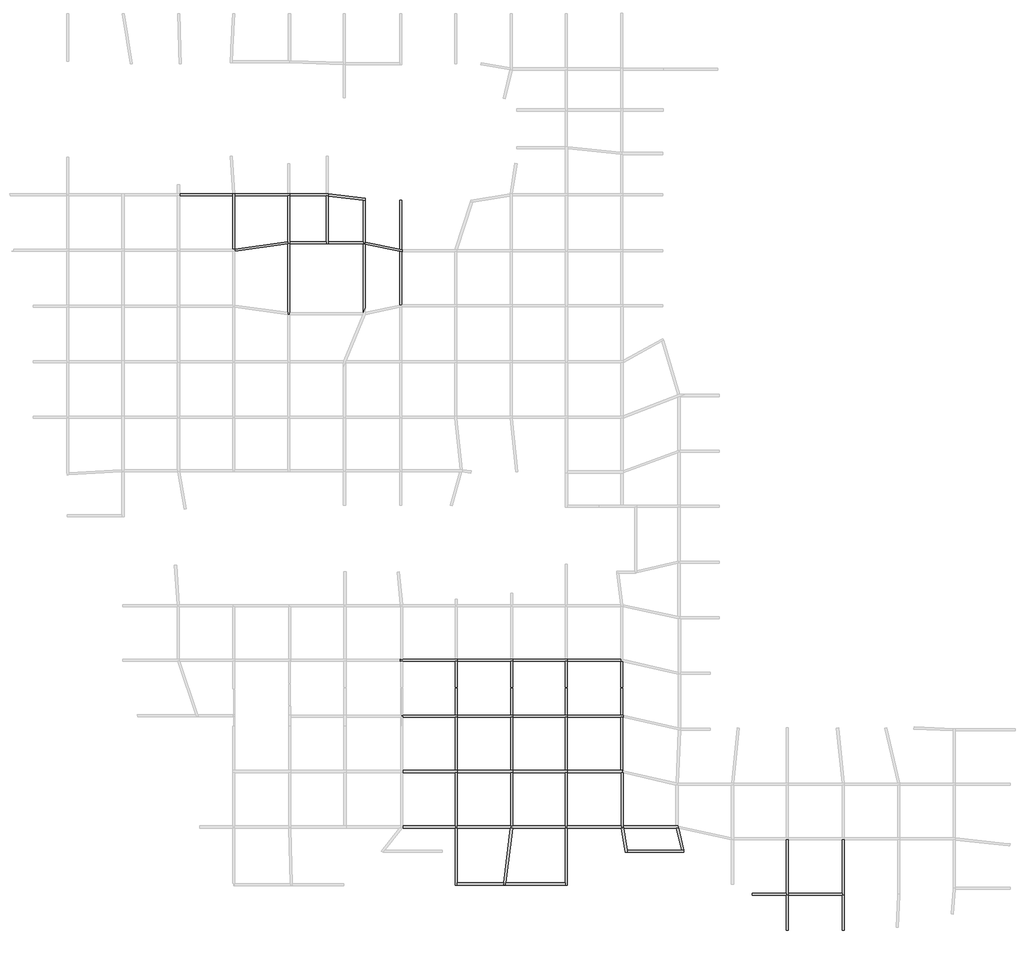
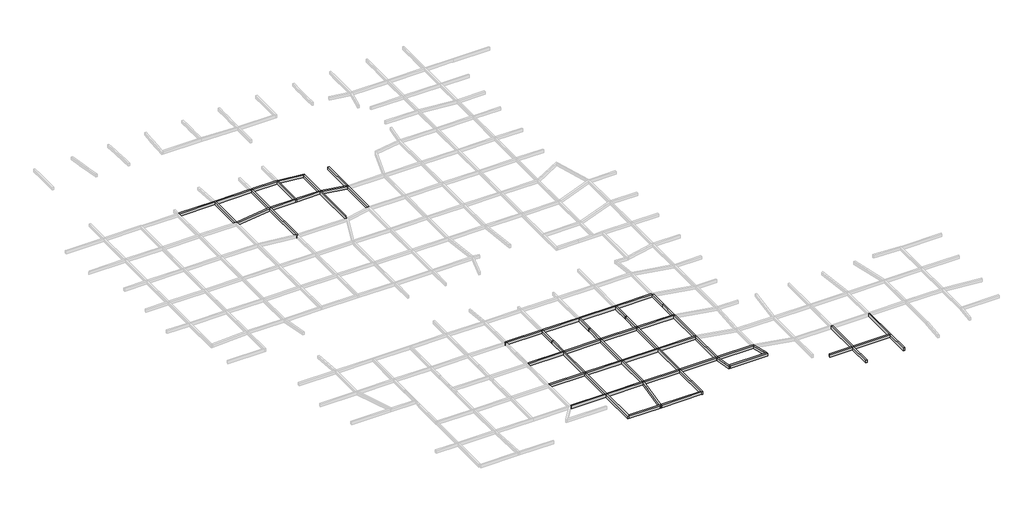
# One storey, part 3 of 8: 59 beams.
"""IFC4 building model written with IfcOpenShell, lengths in millimetres."""

from ifc_helpers import new_model, si_unit, frame, origin, place, context, project, spatial, polyline, outline, extrude, faceted_brep, element, save

model = new_model("IFC4")

# Units and contexts
model_context = context("Model", 3, world=origin())
ifc_project = project(units=[si_unit("LENGTHUNIT", "METRE", prefix="MILLI")], contexts=[model_context])

# Site, building, storey
site = spatial("IfcSite", under=ifc_project)
building = spatial("IfcBuilding", under=site)
storey = spatial("IfcBuildingStorey", under=building, Name="层高", Elevation=3300.0)

# Beams
placement = place(None, origin())
element("IfcBeam", 1, ObjectType="混凝土 - 矩形梁 : KL_beam", at=placement, inside=storey, context=model_context, shape_type="Brep", body=[
    faceted_brep([(101970.8225114, 127335.802002, 3300.0), (101960.6997743, 127335.802002, 3300.0), (101670.8225114, 127335.802002, 3300.0), (101670.8225114, 127035.802002, 3300.0), (101670.8225114, 119435.802002, 3300.0), (101970.8225114, 119435.802002, 3300.0), (101970.8225114, 119458.440122, 3300.0), (101970.8225114, 127035.802002, 3300.0), (101970.8225114, 127191.0401174, 3300.0), (101970.8225114, 127335.802002, 2700.0), (101970.8225114, 119435.802002, 2700.0), (101970.8225114, 119458.440122, 2700.0), (101970.8225114, 127035.802002, 2700.0), (101970.8225114, 127191.0401174, 2700.0), (101670.8225114, 127335.802002, 2700.0), (101960.6997743, 127335.802002, 2700.0), (101670.8225114, 119435.802002, 2700.0), (101670.8225114, 127035.802002, 2700.0)], [[[0, 1, 2, 3, 4, 5, 6, 7, 8]], [[9, 0, 8, 7, 6, 5, 10, 11, 12, 13]], [[14, 15, 9, 13, 12, 11, 10, 16, 17]], [[2, 14, 17, 16, 4, 3]], [[5, 4, 16, 10]], [[2, 1, 0, 9, 15, 14]]]),
])
element("IfcBeam", 2, ObjectType="混凝土 - 矩形梁 : KL_beam", at=placement, inside=storey, context=model_context, shape_type="Brep", body=[
    faceted_brep([(94070.8225114, 127335.802002, 3300.0), (94070.8225114, 127035.802002, 3300.0), (101670.8225114, 127035.802002, 3300.0), (101670.8225114, 127335.802002, 3300.0), (101659.9672049, 127335.802002, 3300.0), (94070.8225114, 127035.802002, 2700.0), (101670.8225114, 127035.802002, 2700.0), (94070.8225114, 127335.802002, 2700.0), (101659.9672049, 127335.802002, 2700.0), (101670.8225114, 127335.802002, 2700.0)], [[[0, 1, 2, 3, 4]], [[1, 5, 6, 2]], [[5, 7, 8, 9, 6]], [[7, 0, 4, 3, 9, 8]], [[1, 0, 7, 5]], [[3, 2, 6, 9]]]),
])
element("IfcBeam", 3, ObjectType="混凝土 - 矩形梁 : KL_beam", at=placement, inside=storey, context=model_context, shape_type="Brep", body=[
    faceted_brep([(109770.8225114, 127035.802002, 3300.0), (109770.8225114, 127335.802002, 3300.0), (109470.8225114, 127335.802002, 3300.0), (101970.8225114, 127335.802002, 3300.0), (101970.8225114, 127191.0401174, 3300.0), (101981.6778179, 127035.802002, 3300.0), (109470.8225114, 127035.802002, 3300.0), (109770.8225114, 127035.802002, 2700.0), (101981.6778179, 127035.802002, 2700.0), (109470.8225114, 127035.802002, 2700.0), (109770.8225114, 127335.802002, 2700.0), (101970.8225114, 127191.0401174, 2700.0), (101970.8225114, 127335.802002, 2700.0), (109470.8225114, 127335.802002, 2700.0)], [[[0, 1, 2, 3, 4, 5, 6]], [[7, 0, 6, 5, 8, 9]], [[10, 7, 9, 8, 11, 12, 13]], [[12, 3, 2, 1, 10, 13]], [[3, 12, 11, 4]], [[5, 4, 11, 8]], [[1, 0, 7, 10]]]),
])
element("IfcBeam", 4, ObjectType="混凝土 - 矩形梁 : KL_beam", at=placement, inside=storey, context=model_context, shape_type="Brep", body=[
    faceted_brep([(115273.8238915, 127035.802002, 3300.0), (115273.8238915, 127318.5107917, 3300.0), (115273.8238915, 127335.802002, 3300.0), (114973.8238915, 127335.802002, 3300.0), (109770.8225114, 127335.802002, 3300.0), (109770.8225114, 127035.802002, 3300.0), (114973.8238915, 127035.802002, 3300.0), (115114.6494985, 127035.802002, 3300.0), (115273.8238915, 127035.802002, 2700.0), (109770.8225114, 127035.802002, 2700.0), (114973.8238915, 127035.802002, 2700.0), (115114.6494985, 127035.802002, 2700.0), (115273.8238915, 127335.802002, 2700.0), (115273.8238915, 127318.5107917, 2700.0), (109770.8225114, 127335.802002, 2700.0), (114973.8238915, 127335.802002, 2700.0)], [[[0, 1, 2, 3, 4, 5, 6, 7]], [[8, 0, 7, 6, 5, 9, 10, 11]], [[12, 13, 8, 11, 10, 9, 14, 15]], [[2, 12, 15, 14, 4, 3]], [[5, 4, 14, 9]], [[2, 1, 0, 8, 13, 12]]]),
])
element("IfcBeam", 5, ObjectType="混凝土 - 矩形梁 : KL_beam", at=placement, inside=storey, context=model_context, shape_type="Brep", body=[
    faceted_brep([(115273.8238915, 127035.802002, 3300.0), (115114.6494985, 127035.802002, 3300.0), (115273.8238915, 127016.2578441, 3300.0), (120234.3184952, 126407.1856923, 3300.0), (120534.3184952, 126370.350324, 3300.0), (120534.3184952, 126672.6032717, 3300.0), (115273.8238915, 127318.5107917, 3300.0), (115114.6494985, 127035.802002, 2700.0), (115273.8238915, 127016.2578441, 2700.0), (120234.3184952, 126407.1856923, 2700.0), (120534.3184952, 126370.350324, 2700.0), (115273.8238915, 127035.802002, 2700.0), (115273.8238915, 127318.5107917, 2700.0), (120534.3184952, 126672.6032717, 2700.0)], [[[0, 1, 2, 3, 4, 5, 6]], [[1, 7, 8, 9, 10, 4, 3, 2]], [[7, 11, 12, 13, 10, 9, 8]], [[12, 6, 5, 13]], [[0, 11, 7, 1]], [[11, 0, 6, 12]], [[5, 4, 10, 13]]]),
])
element("IfcBeam", 6, ObjectType="混凝土 - 矩形梁 : KL_beam", at=placement, inside=storey, context=model_context, shape_type="Brep", body=[
    faceted_brep([(109470.8225114, 120235.802002, 3300.0), (109770.8225114, 120235.802002, 3300.0), (109770.8225114, 120535.802002, 3300.0), (109770.8225114, 127035.802002, 3300.0), (109470.8225114, 127035.802002, 3300.0), (109470.8225114, 120516.1324297, 3300.0), (109470.8225114, 120235.802002, 2700.0), (109470.8225114, 127035.802002, 2700.0), (109470.8225114, 120516.1324297, 2700.0), (109770.8225114, 120235.802002, 2700.0), (109770.8225114, 127035.802002, 2700.0), (109770.8225114, 120535.802002, 2700.0)], [[[0, 1, 2, 3, 4, 5]], [[6, 0, 5, 4, 7, 8]], [[9, 6, 8, 7, 10, 11]], [[1, 9, 11, 10, 3, 2]], [[4, 3, 10, 7]], [[1, 0, 6, 9]]]),
])
element("IfcBeam", 7, ObjectType="混凝土 - 矩形梁 : KL_beam", at=placement, inside=storey, context=model_context, shape_type="Brep", body=[
    faceted_brep([(109470.8225114, 110106.8473936, 3300.0), (109770.8225114, 110106.8473936, 3300.0), (109770.8225114, 110406.8473936, 3300.0), (109770.8225114, 120235.802002, 3300.0), (109470.8225114, 120235.802002, 3300.0), (109470.8225114, 120213.1638821, 3300.0), (109470.8225114, 110428.8334253, 3300.0), (109470.8225114, 110126.0228157, 3300.0), (109470.8225114, 110106.8473936, 2700.0), (109470.8225114, 120235.802002, 2700.0), (109470.8225114, 120213.1638821, 2700.0), (109470.8225114, 110428.8334253, 2700.0), (109470.8225114, 110126.0228157, 2700.0), (109770.8225114, 110106.8473936, 2700.0), (109770.8225114, 120235.802002, 2700.0), (109770.8225114, 110406.8473936, 2700.0)], [[[0, 1, 2, 3, 4, 5, 6, 7]], [[8, 0, 7, 6, 5, 4, 9, 10, 11, 12]], [[13, 8, 12, 11, 10, 9, 14, 15]], [[1, 13, 15, 14, 3, 2]], [[4, 3, 14, 9]], [[1, 0, 8, 13]]]),
])
element("IfcBeam", 8, ObjectType="混凝土 - 矩形梁 : KL_beam", at=placement, inside=storey, context=model_context, shape_type="Brep", body=[
    faceted_brep([(114973.8238915, 120235.802002, 3300.0), (115273.8238915, 120235.802002, 3300.0), (115273.8238915, 120535.802002, 3300.0), (115273.8238915, 127016.2578441, 3300.0), (115114.6494985, 127035.802002, 3300.0), (114973.8238915, 127035.802002, 3300.0), (114973.8238915, 120535.802002, 3300.0), (114973.8238915, 127035.802002, 2700.0), (114973.8238915, 120535.802002, 2700.0), (114973.8238915, 120235.802002, 2700.0), (115273.8238915, 120235.802002, 2700.0), (115114.6494985, 127035.802002, 2700.0), (115273.8238915, 127016.2578441, 2700.0), (115273.8238915, 120535.802002, 2700.0)], [[[0, 1, 2, 3, 4, 5, 6]], [[5, 7, 8, 9, 0, 6]], [[10, 9, 8, 7, 11, 12, 13]], [[1, 10, 13, 12, 3, 2]], [[7, 5, 4, 11]], [[4, 3, 12, 11]], [[1, 0, 9, 10]]]),
])
element("IfcBeam", 9, ObjectType="混凝土 - 矩形梁 : KL_beam", at=placement, inside=storey, context=model_context, shape_type="Brep", body=[
    faceted_brep([(120234.3184952, 120235.802002, 3300.0), (120534.3184952, 120235.802002, 3300.0), (120534.3184952, 120466.4709981, 3300.0), (120534.3184952, 126370.350324, 3300.0), (120234.3184952, 126407.1856923, 3300.0), (120234.3184952, 120535.802002, 3300.0), (120234.3184952, 120235.802002, 2700.0), (120234.3184952, 126407.1856923, 2700.0), (120234.3184952, 120535.802002, 2700.0), (120534.3184952, 120235.802002, 2700.0), (120534.3184952, 126370.350324, 2700.0), (120534.3184952, 120466.4709981, 2700.0)], [[[0, 1, 2, 3, 4, 5]], [[6, 0, 5, 4, 7, 8]], [[9, 6, 8, 7, 10, 11]], [[1, 9, 11, 10, 3, 2]], [[4, 3, 10, 7]], [[1, 0, 6, 9]]]),
])
element("IfcBeam", 10, ObjectType="混凝土 - 矩形梁 : KL_beam", at=placement, inside=storey, context=model_context, shape_type="SweptSolid", body=[
    extrude(outline(polyline([(109770.8225114, 120235.802002), (109770.8225114, 120535.802002), (114973.8238915, 120535.802002), (114973.8238915, 120235.802002), (109770.8225114, 120235.802002)])), frame((0.0, 0.0, 2700.0), z_axis=(0.0, 0.0, 1.0), x_axis=(1.0, 0.0, 0.0)), (0.0, 0.0, 1.0), 600.0),
])
element("IfcBeam", 11, ObjectType="混凝土 - 矩形梁 : KL_beam", at=placement, inside=storey, context=model_context, shape_type="SweptSolid", body=[
    extrude(outline(polyline([(115273.8238915, 120235.802002), (115273.8238915, 120535.802002), (120234.3184952, 120535.802002), (120234.3184952, 120235.802002), (115273.8238915, 120235.802002)])), frame((0.0, 0.0, 2700.0), z_axis=(0.0, 0.0, 1.0), x_axis=(1.0, 0.0, 0.0)), (0.0, 0.0, 1.0), 600.0),
])
element("IfcBeam", 12, ObjectType="混凝土 - 矩形梁 : KL_beam", at=placement, inside=storey, context=model_context, shape_type="Brep", body=[
    faceted_brep([(120234.3184952, 110286.2989162, 3300.0), (120534.3184952, 111020.8146845, 3300.0), (120534.3184952, 120159.7688197, 3300.0), (120234.3184952, 120223.5357882, 3300.0), (120234.3184952, 110406.8473936, 3300.0), (120234.3184952, 110286.2989162, 2700.0), (120234.3184952, 120223.5357882, 2700.0), (120234.3184952, 110406.8473936, 2700.0), (120534.3184952, 111020.8146845, 2700.0), (120534.3184952, 120159.7688197, 2700.0)], [[[0, 1, 2, 3, 4]], [[5, 0, 4, 3, 6, 7]], [[8, 5, 7, 6, 9]], [[1, 8, 9, 2]], [[1, 0, 5, 8]], [[3, 2, 9, 6]]]),
])
element("IfcBeam", 13, ObjectType="混凝土 - 矩形梁 : KL_beam", at=placement, inside=storey, context=model_context, shape_type="Brep", body=[
    faceted_brep([(120234.3184952, 120223.5357882, 3300.0), (120534.3184952, 120159.7688197, 3300.0), (125448.8238726, 119115.1584543, 3300.0), (125748.8238726, 119051.3914858, 3300.0), (125783.0582452, 119044.1147453, 3300.0), (125814.5895158, 119344.1147453, 3300.0), (125748.8238726, 119358.0936643, 3300.0), (125448.8238726, 119421.8606328, 3300.0), (120534.3184952, 120466.4709981, 3300.0), (120534.3184952, 120235.802002, 3300.0), (120234.3184952, 120235.802002, 3300.0), (120234.3184952, 120223.5357882, 2700.0), (120534.3184952, 120159.7688197, 2700.0), (125448.8238726, 119115.1584543, 2700.0), (125748.8238726, 119051.3914858, 2700.0), (125783.0582452, 119044.1147453, 2700.0), (120234.3184952, 120235.802002, 2700.0), (120534.3184952, 120235.802002, 2700.0), (120534.3184952, 120466.4709981, 2700.0), (125448.8238726, 119421.8606328, 2700.0), (125748.8238726, 119358.0936643, 2700.0), (125814.5895158, 119344.1147453, 2700.0)], [[[0, 1, 2, 3, 4, 5, 6, 7, 8, 9, 10]], [[4, 3, 2, 1, 0, 11, 12, 13, 14, 15]], [[15, 14, 13, 12, 11, 16, 17, 18, 19, 20, 21]], [[8, 7, 6, 5, 21, 20, 19, 18]], [[11, 0, 10, 16]], [[9, 17, 16, 10]], [[17, 9, 8, 18]], [[5, 4, 15, 21]]]),
])
element("IfcBeam", 14, ObjectType="混凝土 - 矩形梁 : KL_beam", at=placement, inside=storey, context=model_context, shape_type="SweptSolid", body=[
    extrude(outline(polyline([(125748.8238726, 111550.4593009), (125448.8238726, 111486.6923324), (125448.8238726, 119115.1584543), (125748.8238726, 119051.3914858), (125748.8238726, 111550.4593009)])), frame((0.0, 0.0, 2700.0), z_axis=(0.0, 0.0, 1.0), x_axis=(1.0, 0.0, 0.0)), (0.0, 0.0, 1.0), 600.0),
])
element("IfcBeam", 15, ObjectType="混凝土 - 矩形梁 : KL_beam", at=placement, inside=storey, context=model_context, shape_type="SweptSolid", body=[
    extrude(outline(polyline([(125448.8238726, 126395.9353335), (125748.8238726, 126395.9353335), (125748.8238726, 119358.0936643), (125448.8238726, 119421.8606328), (125448.8238726, 126395.9353335)])), frame((0.0, 0.0, 2700.0), z_axis=(0.0, 0.0, 1.0), x_axis=(1.0, 0.0, 0.0)), (0.0, 0.0, 1.0), 600.0),
])
element("IfcBeam", 16, ObjectType="混凝土 - 矩形梁 : KL_beam", at=placement, inside=storey, context=model_context, shape_type="Brep", body=[
    faceted_brep([(156926.4248507, 53082.6668088, 3300.0), (157226.4248507, 53082.6668088, 3300.0), (157226.4248507, 56907.0370398, 3300.0), (156926.4248507, 56907.0370398, 3300.0), (156926.4248507, 53082.6668088, 2700.0), (156926.4248507, 56907.0370398, 2700.0), (157226.4248507, 53082.6668088, 2700.0), (157226.4248507, 56907.0370398, 2700.0)], [[[0, 1, 2, 3]], [[4, 0, 3, 5]], [[6, 4, 5, 7]], [[1, 6, 7, 2]], [[1, 0, 4, 6]], [[3, 2, 7, 5]]]),
    faceted_brep([(156926.4248507, 60756.0063653, 3300.0), (157226.4248507, 60688.1226811, 3300.0), (157226.4248507, 60688.1226811, 2700.0), (156926.4248507, 60756.0063653, 2700.0), (157226.4248507, 57027.0370398, 3300.0), (156926.4248507, 57027.0370398, 3300.0), (156926.4248507, 57027.0370398, 2700.0), (157226.4248507, 57027.0370398, 2700.0), (156926.4248507, 60727.1438632, 3300.0), (156926.4248507, 60727.1438632, 2700.0)], [[[0, 1, 2, 3]], [[4, 5, 6, 7]], [[1, 0, 8, 5, 4]], [[0, 3, 9, 6, 5, 8]], [[3, 2, 7, 6, 9]], [[2, 1, 4, 7]]]),
])
element("IfcBeam", 17, ObjectType="混凝土 - 矩形梁 : KL_beam", at=placement, inside=storey, context=model_context, shape_type="Brep", body=[
    faceted_brep([(125476.4248507, 61027.1438632, 3300.0), (125476.4248507, 60727.1438632, 3300.0), (125548.8240412, 60727.1438632, 3300.0), (125848.8240412, 60727.1438632, 3300.0), (133326.4248507, 60727.1438632, 3300.0), (133626.4248507, 60727.1438632, 3300.0), (133626.4248507, 61027.1438632, 3300.0), (133326.4248507, 61027.1438632, 3300.0), (125848.8240412, 61027.1438632, 3300.0), (125548.8240412, 61027.1438632, 3300.0), (125476.4248507, 60727.1438632, 2700.0), (125548.8240412, 60727.1438632, 2700.0), (125848.8240412, 60727.1438632, 2700.0), (133326.4248507, 60727.1438632, 2700.0), (133626.4248507, 60727.1438632, 2700.0), (125476.4248507, 61027.1438632, 2700.0), (125548.8240412, 61027.1438632, 2700.0), (125848.8240412, 61027.1438632, 2700.0), (133326.4248507, 61027.1438632, 2700.0), (133626.4248507, 61027.1438632, 2700.0)], [[[0, 1, 2, 3, 4, 5, 6, 7, 8, 9]], [[1, 10, 11, 12, 13, 14, 5, 4, 3, 2]], [[10, 15, 16, 17, 18, 19, 14, 13, 12, 11]], [[15, 0, 9, 8, 7, 6, 19, 18, 17, 16]], [[0, 15, 10, 1]], [[6, 5, 14, 19]]]),
])
element("IfcBeam", 18, ObjectType="混凝土 - 矩形梁 : KL_beam", at=placement, inside=storey, context=model_context, shape_type="Brep", body=[
    faceted_brep([(141526.4248507, 60727.1438632, 3300.0), (141526.4248507, 61027.1438632, 3300.0), (141226.4248507, 61027.1438632, 3300.0), (133626.4248507, 61027.1438632, 3300.0), (133626.4248507, 60727.1438632, 3300.0), (141226.4248507, 60727.1438632, 3300.0), (141526.4248507, 60727.1438632, 2700.0), (133626.4248507, 60727.1438632, 2700.0), (141226.4248507, 60727.1438632, 2700.0), (141526.4248507, 61027.1438632, 2700.0), (133626.4248507, 61027.1438632, 2700.0), (141226.4248507, 61027.1438632, 2700.0)], [[[0, 1, 2, 3, 4, 5]], [[6, 0, 5, 4, 7, 8]], [[9, 6, 8, 7, 10, 11]], [[1, 9, 11, 10, 3, 2]], [[4, 3, 10, 7]], [[1, 0, 6, 9]]]),
])
element("IfcBeam", 19, ObjectType="混凝土 - 矩形梁 : KL_beam", at=placement, inside=storey, context=model_context, shape_type="Brep", body=[
    faceted_brep([(149326.4248507, 60727.1438632, 3300.0), (149326.4248507, 61027.1438632, 3300.0), (149026.4248507, 61027.1438632, 3300.0), (141526.4248507, 61027.1438632, 3300.0), (141526.4248507, 60727.1438632, 3300.0), (149026.4248507, 60727.1438632, 3300.0), (149326.4248507, 60727.1438632, 2700.0), (141526.4248507, 60727.1438632, 2700.0), (149026.4248507, 60727.1438632, 2700.0), (149326.4248507, 61027.1438632, 2700.0), (141526.4248507, 61027.1438632, 2700.0), (149026.4248507, 61027.1438632, 2700.0)], [[[0, 1, 2, 3, 4, 5]], [[6, 0, 5, 4, 7, 8]], [[9, 6, 8, 7, 10, 11]], [[1, 9, 11, 10, 3, 2]], [[1, 0, 6, 9]], [[4, 3, 10, 7]]]),
])
element("IfcBeam", 20, ObjectType="混凝土 - 矩形梁 : KL_beam", at=placement, inside=storey, context=model_context, shape_type="Brep", body=[
    faceted_brep([(156926.4248507, 60727.1438632, 3300.0), (156926.4248507, 60756.0063653, 3300.0), (156926.4248507, 61027.1438632, 3300.0), (149326.4248507, 61027.1438632, 3300.0), (149326.4248507, 60727.1438632, 3300.0), (149326.4248507, 60727.1438632, 2700.0), (156926.4248507, 60727.1438632, 2700.0), (156926.4248507, 61027.1438632, 2700.0), (156926.4248507, 60756.0063653, 2700.0), (149326.4248507, 61027.1438632, 2700.0)], [[[0, 1, 2, 3, 4]], [[4, 5, 6, 0]], [[7, 8, 6, 5, 9]], [[2, 7, 9, 3]], [[0, 6, 8, 7, 2, 1]], [[4, 3, 9, 5]]]),
])
element("IfcBeam", 21, ObjectType="混凝土 - 矩形梁 : KL_beam", at=placement, inside=storey, context=model_context, shape_type="Brep", body=[
    faceted_brep([(133626.4248507, 52782.6668088, 3300.0), (133626.4248507, 53082.6668088, 3300.0), (133326.4248507, 53082.6668088, 3300.0), (125848.8240412, 53082.6668088, 3300.0), (125758.8240412, 53082.6668088, 3300.0), (125758.8240412, 52932.6668088, 3300.0), (125848.8240412, 52932.6668088, 3300.0), (125848.8240412, 52782.6668088, 3300.0), (133326.4248507, 52782.6668088, 3300.0), (133626.4248507, 52782.6668088, 2700.0), (125848.8240412, 52782.6668088, 2700.0), (133326.4248507, 52782.6668088, 2700.0), (133626.4248507, 53082.6668088, 2700.0), (125848.8240412, 52932.6668088, 2700.0), (125758.8240412, 52932.6668088, 2700.0), (125758.8240412, 53082.6668088, 2700.0), (125848.8240412, 53082.6668088, 2700.0), (133326.4248507, 53082.6668088, 2700.0)], [[[0, 1, 2, 3, 4, 5, 6, 7, 8]], [[9, 0, 8, 7, 10, 11]], [[12, 9, 11, 10, 13, 14, 15, 16, 17]], [[1, 12, 17, 16, 15, 4, 3, 2]], [[6, 13, 10, 7]], [[1, 0, 9, 12]], [[4, 15, 14, 5]], [[13, 6, 5, 14]]]),
])
element("IfcBeam", 22, ObjectType="混凝土 - 矩形梁 : KL_beam", at=placement, inside=storey, context=model_context, shape_type="Brep", body=[
    faceted_brep([(141526.4248507, 52782.6668088, 3300.0), (141526.4248507, 53082.6668088, 3300.0), (141226.4248507, 53082.6668088, 3300.0), (133626.4248507, 53082.6668088, 3300.0), (133626.4248507, 52782.6668088, 3300.0), (141226.4248507, 52782.6668088, 3300.0), (141526.4248507, 52782.6668088, 2700.0), (133626.4248507, 52782.6668088, 2700.0), (141226.4248507, 52782.6668088, 2700.0), (141526.4248507, 53082.6668088, 2700.0), (133626.4248507, 53082.6668088, 2700.0), (141226.4248507, 53082.6668088, 2700.0)], [[[0, 1, 2, 3, 4, 5]], [[6, 0, 5, 4, 7, 8]], [[9, 6, 8, 7, 10, 11]], [[1, 9, 11, 10, 3, 2]], [[4, 3, 10, 7]], [[1, 0, 6, 9]]]),
])
element("IfcBeam", 23, ObjectType="混凝土 - 矩形梁 : KL_beam", at=placement, inside=storey, context=model_context, shape_type="Brep", body=[
    faceted_brep([(149326.4248507, 52782.6668088, 3300.0), (149326.4248507, 53082.6668088, 3300.0), (149026.4248507, 53082.6668088, 3300.0), (141526.4248507, 53082.6668088, 3300.0), (141526.4248507, 52782.6668088, 3300.0), (149026.4248507, 52782.6668088, 3300.0), (149326.4248507, 52782.6668088, 2700.0), (141526.4248507, 52782.6668088, 2700.0), (149026.4248507, 52782.6668088, 2700.0), (149326.4248507, 53082.6668088, 2700.0), (141526.4248507, 53082.6668088, 2700.0), (149026.4248507, 53082.6668088, 2700.0)], [[[0, 1, 2, 3, 4, 5]], [[6, 0, 5, 4, 7, 8]], [[9, 6, 8, 7, 10, 11]], [[1, 9, 11, 10, 3, 2]], [[4, 3, 10, 7]], [[1, 0, 6, 9]]]),
])
element("IfcBeam", 24, ObjectType="混凝土 - 矩形梁 : KL_beam", at=placement, inside=storey, context=model_context, shape_type="Brep", body=[
    faceted_brep([(149326.4248507, 53082.6668088, 3300.0), (149326.4248507, 52782.6668088, 3300.0), (156926.4248507, 52782.6668088, 3300.0), (157226.4248507, 52782.6668088, 3300.0), (157246.4106924, 52782.6668088, 3300.0), (157280.5913749, 53082.6668088, 3300.0), (157226.4248507, 53082.6668088, 3300.0), (156926.4248507, 53082.6668088, 3300.0), (149326.4248507, 52782.6668088, 2700.0), (156926.4248507, 52782.6668088, 2700.0), (157226.4248507, 52782.6668088, 2700.0), (157246.4106924, 52782.6668088, 2700.0), (149326.4248507, 53082.6668088, 2700.0), (156926.4248507, 53082.6668088, 2700.0), (157226.4248507, 53082.6668088, 2700.0), (157280.5913749, 53082.6668088, 2700.0)], [[[0, 1, 2, 3, 4, 5, 6, 7]], [[1, 8, 9, 10, 11, 4, 3, 2]], [[8, 12, 13, 14, 15, 11, 10, 9]], [[12, 0, 7, 6, 5, 15, 14, 13]], [[1, 0, 12, 8]], [[5, 4, 11, 15]]]),
])
element("IfcBeam", 25, ObjectType="混凝土 - 矩形梁 : KL_beam", at=placement, inside=storey, context=model_context, shape_type="Brep", body=[
    faceted_brep([(133626.4248507, 44882.6668088, 3300.0), (133626.4248507, 45182.6668088, 3300.0), (133326.4248507, 45182.6668088, 3300.0), (125848.8240412, 45182.6668088, 3300.0), (125848.8240412, 44882.6668088, 3300.0), (133326.4248507, 44882.6668088, 3300.0), (133626.4248507, 44882.6668088, 2700.0), (125848.8240412, 44882.6668088, 2700.0), (133326.4248507, 44882.6668088, 2700.0), (133626.4248507, 45182.6668088, 2700.0), (125848.8240412, 45182.6668088, 2700.0), (133326.4248507, 45182.6668088, 2700.0)], [[[0, 1, 2, 3, 4, 5]], [[6, 0, 5, 4, 7, 8]], [[9, 6, 8, 7, 10, 11]], [[1, 9, 11, 10, 3, 2]], [[4, 3, 10, 7]], [[1, 0, 6, 9]]]),
])
element("IfcBeam", 26, ObjectType="混凝土 - 矩形梁 : KL_beam", at=placement, inside=storey, context=model_context, shape_type="Brep", body=[
    faceted_brep([(141526.4248507, 44882.6668088, 3300.0), (141526.4248507, 45182.6668088, 3300.0), (141226.4248507, 45182.6668088, 3300.0), (133626.4248507, 45182.6668088, 3300.0), (133626.4248507, 44882.6668088, 3300.0), (141226.4248507, 44882.6668088, 3300.0), (141526.4248507, 44882.6668088, 2700.0), (133626.4248507, 44882.6668088, 2700.0), (141226.4248507, 44882.6668088, 2700.0), (141526.4248507, 45182.6668088, 2700.0), (133626.4248507, 45182.6668088, 2700.0), (141226.4248507, 45182.6668088, 2700.0)], [[[0, 1, 2, 3, 4, 5]], [[6, 0, 5, 4, 7, 8]], [[9, 6, 8, 7, 10, 11]], [[1, 9, 11, 10, 3, 2]], [[4, 3, 10, 7]], [[1, 0, 6, 9]]]),
])
element("IfcBeam", 27, ObjectType="混凝土 - 矩形梁 : KL_beam", at=placement, inside=storey, context=model_context, shape_type="Brep", body=[
    faceted_brep([(149326.4248507, 44882.6668088, 3300.0), (149326.4248507, 45182.6668088, 3300.0), (149026.4248507, 45182.6668088, 3300.0), (141526.4248507, 45182.6668088, 3300.0), (141526.4248507, 44882.6668088, 3300.0), (149026.4248507, 44882.6668088, 3300.0), (149326.4248507, 44882.6668088, 2700.0), (141526.4248507, 44882.6668088, 2700.0), (149026.4248507, 44882.6668088, 2700.0), (149326.4248507, 45182.6668088, 2700.0), (141526.4248507, 45182.6668088, 2700.0), (149026.4248507, 45182.6668088, 2700.0)], [[[0, 1, 2, 3, 4, 5]], [[6, 0, 5, 4, 7, 8]], [[9, 6, 8, 7, 10, 11]], [[1, 9, 11, 10, 3, 2]], [[4, 3, 10, 7]], [[1, 0, 6, 9]]]),
])
element("IfcBeam", 28, ObjectType="混凝土 - 矩形梁 : KL_beam", at=placement, inside=storey, context=model_context, shape_type="Brep", body=[
    faceted_brep([(157131.7337266, 44882.6668088, 3300.0), (157165.9144091, 45182.6668088, 3300.0), (156926.4248507, 45182.6668088, 3300.0), (149326.4248507, 45182.6668088, 3300.0), (149326.4248507, 44882.6668088, 3300.0), (156998.8240678, 44882.6668088, 3300.0), (157131.7337266, 44882.6668088, 2700.0), (149326.4248507, 44882.6668088, 2700.0), (156998.8240678, 44882.6668088, 2700.0), (157165.9144091, 45182.6668088, 2700.0), (149326.4248507, 45182.6668088, 2700.0), (156926.4248507, 45182.6668088, 2700.0)], [[[0, 1, 2, 3, 4, 5]], [[6, 0, 5, 4, 7, 8]], [[9, 6, 8, 7, 10, 11]], [[1, 9, 11, 10, 3, 2]], [[1, 0, 6, 9]], [[4, 3, 10, 7]]]),
])
element("IfcBeam", 29, ObjectType="混凝土 - 矩形梁 : KL_beam", at=placement, inside=storey, context=model_context, shape_type="SweptSolid", body=[
    extrude(outline(polyline([(156926.4248507, 52782.6668088), (157226.4248507, 52782.6668088), (157226.4248507, 45168.6968726), (157165.9144091, 45182.6668088), (156926.4248507, 45182.6668088), (156926.4248507, 52782.6668088)])), frame((0.0, 0.0, 2700.0), z_axis=(0.0, 0.0, 1.0), x_axis=(1.0, 0.0, 0.0)), (0.0, 0.0, 1.0), 600.0),
])
element("IfcBeam", 30, ObjectType="混凝土 - 矩形梁 : KL_beam", at=placement, inside=storey, context=model_context, shape_type="Brep", body=[
    faceted_brep([(101970.8225114, 119458.440122, 3300.0), (101970.8225114, 119435.802002, 3300.0), (101970.8225114, 119155.4715744, 3300.0), (109470.8225114, 120213.1638821, 3300.0), (109470.8225114, 120235.802002, 3300.0), (109470.8225114, 120516.1324297, 3300.0), (101970.8225114, 119155.4715744, 2700.0), (109470.8225114, 120213.1638821, 2700.0), (101970.8225114, 119435.802002, 2700.0), (101970.8225114, 119458.440122, 2700.0), (109470.8225114, 120516.1324297, 2700.0), (109470.8225114, 120235.802002, 2700.0)], [[[0, 1, 2, 3, 4, 5]], [[2, 6, 7, 3]], [[6, 8, 9, 10, 11, 7]], [[9, 0, 5, 10]], [[6, 2, 1, 0, 9, 8]], [[3, 7, 11, 10, 5, 4]]]),
])
element("IfcBeam", 31, ObjectType="混凝土 - 矩形梁 : KL_beam", at=placement, inside=storey, context=model_context, shape_type="SweptSolid", body=[
    extrude(outline(polyline([(133626.4248507, 53082.6668088), (133326.4248507, 53082.6668088), (133326.4248507, 56907.0370398), (133626.4248507, 56907.0370398), (133626.4248507, 53082.6668088)])), frame((0.0, 0.0, 2700.0), z_axis=(0.0, 0.0, 1.0), x_axis=(1.0, 0.0, 0.0)), (0.0, 0.0, 1.0), 600.0),
    extrude(outline(polyline([(133326.4248507, 60727.1438632), (133626.4248507, 60727.1438632), (133626.4248507, 57027.0370398), (133326.4248507, 57027.0370398), (133326.4248507, 60727.1438632)])), frame((0.0, 0.0, 2700.0), z_axis=(0.0, 0.0, 1.0), x_axis=(1.0, 0.0, 0.0)), (0.0, 0.0, 1.0), 600.0),
])
element("IfcBeam", 32, ObjectType="混凝土 - 矩形梁 : KL_beam", at=placement, inside=storey, context=model_context, shape_type="SweptSolid", body=[
    extrude(outline(polyline([(133326.4248507, 52782.6668088), (133626.4248507, 52782.6668088), (133626.4248507, 45182.6668088), (133326.4248507, 45182.6668088), (133326.4248507, 52782.6668088)])), frame((0.0, 0.0, 2700.0), z_axis=(0.0, 0.0, 1.0), x_axis=(1.0, 0.0, 0.0)), (0.0, 0.0, 1.0), 600.0),
])
element("IfcBeam", 33, ObjectType="混凝土 - 矩形梁 : KL_beam", at=placement, inside=storey, context=model_context, shape_type="SweptSolid", body=[
    extrude(outline(polyline([(141526.4248507, 53082.6668088), (141226.4248507, 53082.6668088), (141226.4248507, 56907.0370398), (141526.4248507, 56907.0370398), (141526.4248507, 53082.6668088)])), frame((0.0, 0.0, 2700.0), z_axis=(0.0, 0.0, 1.0), x_axis=(1.0, 0.0, 0.0)), (0.0, 0.0, 1.0), 600.0),
    extrude(outline(polyline([(141226.4248507, 60727.1438632), (141526.4248507, 60727.1438632), (141526.4248507, 57027.0370398), (141226.4248507, 57027.0370398), (141226.4248507, 60727.1438632)])), frame((0.0, 0.0, 2700.0), z_axis=(0.0, 0.0, 1.0), x_axis=(1.0, 0.0, 0.0)), (0.0, 0.0, 1.0), 600.0),
])
element("IfcBeam", 34, ObjectType="混凝土 - 矩形梁 : KL_beam", at=placement, inside=storey, context=model_context, shape_type="SweptSolid", body=[
    extrude(outline(polyline([(141226.4248507, 52782.6668088), (141526.4248507, 52782.6668088), (141526.4248507, 45182.6668088), (141226.4248507, 45182.6668088), (141226.4248507, 52782.6668088)])), frame((0.0, 0.0, 2700.0), z_axis=(0.0, 0.0, 1.0), x_axis=(1.0, 0.0, 0.0)), (0.0, 0.0, 1.0), 600.0),
])
element("IfcBeam", 35, ObjectType="混凝土 - 矩形梁 : KL_beam", at=placement, inside=storey, context=model_context, shape_type="SweptSolid", body=[
    extrude(outline(polyline([(149326.4248507, 53082.6668088), (149026.4248507, 53082.6668088), (149026.4248507, 56907.0370398), (149326.4248507, 56907.0370398), (149326.4248507, 53082.6668088)])), frame((0.0, 0.0, 2700.0), z_axis=(0.0, 0.0, 1.0), x_axis=(1.0, 0.0, 0.0)), (0.0, 0.0, 1.0), 600.0),
    extrude(outline(polyline([(149026.4248507, 60727.1438632), (149326.4248507, 60727.1438632), (149326.4248507, 57027.0370398), (149026.4248507, 57027.0370398), (149026.4248507, 60727.1438632)])), frame((0.0, 0.0, 2700.0), z_axis=(0.0, 0.0, 1.0), x_axis=(1.0, 0.0, 0.0)), (0.0, 0.0, 1.0), 600.0),
])
element("IfcBeam", 36, ObjectType="混凝土 - 矩形梁 : KL_beam", at=placement, inside=storey, context=model_context, shape_type="SweptSolid", body=[
    extrude(outline(polyline([(149026.4248507, 52782.6668088), (149326.4248507, 52782.6668088), (149326.4248507, 45182.6668088), (149026.4248507, 45182.6668088), (149026.4248507, 52782.6668088)])), frame((0.0, 0.0, 2700.0), z_axis=(0.0, 0.0, 1.0), x_axis=(1.0, 0.0, 0.0)), (0.0, 0.0, 1.0), 600.0),
])
element("IfcBeam", 37, ObjectType="混凝土 - 矩形梁 : KL_beam", at=placement, inside=storey, context=model_context, shape_type="Brep", body=[
    faceted_brep([(149026.4248507, 36982.6668088, 3300.0), (149326.4248507, 36982.6668088, 3300.0), (149326.4248507, 37282.6668088, 3300.0), (149326.4248507, 44882.6668088, 3300.0), (149026.4248507, 44882.6668088, 3300.0), (149026.4248507, 37282.6668088, 3300.0), (149026.4248507, 36982.6668088, 2700.0), (149026.4248507, 44882.6668088, 2700.0), (149026.4248507, 37282.6668088, 2700.0), (149326.4248507, 36982.6668088, 2700.0), (149326.4248507, 44882.6668088, 2700.0), (149326.4248507, 37282.6668088, 2700.0)], [[[0, 1, 2, 3, 4, 5]], [[6, 0, 5, 4, 7, 8]], [[9, 6, 8, 7, 10, 11]], [[1, 9, 11, 10, 3, 2]], [[4, 3, 10, 7]], [[1, 0, 6, 9]]]),
])
element("IfcBeam", 38, ObjectType="混凝土 - 矩形梁 : KL_beam", at=placement, inside=storey, context=model_context, shape_type="Brep", body=[
    faceted_brep([(149026.4248507, 28855.6854093, 3300.0), (149326.4248507, 28855.6854093, 3300.0), (149326.4248507, 36982.6668088, 3300.0), (149026.4248507, 36982.6668088, 3300.0), (149026.4248507, 29155.6854093, 3300.0), (149026.4248507, 28855.6854093, 2700.0), (149026.4248507, 36982.6668088, 2700.0), (149026.4248507, 29155.6854093, 2700.0), (149326.4248507, 28855.6854093, 2700.0), (149326.4248507, 36982.6668088, 2700.0)], [[[0, 1, 2, 3, 4]], [[5, 0, 4, 3, 6, 7]], [[8, 5, 7, 6, 9]], [[1, 8, 9, 2]], [[3, 2, 9, 6]], [[1, 0, 5, 8]]]),
])
element("IfcBeam", 39, ObjectType="混凝土 - 矩形梁 : KL_beam", at=placement, inside=storey, context=model_context, shape_type="Brep", body=[
    faceted_brep([(157131.7337266, 44882.6668088, 3300.0), (156998.8240678, 44882.6668088, 3300.0), (156998.8240678, 37282.6668088, 3300.0), (156998.8240678, 36982.6668088, 3300.0), (157020.711965, 36982.6668088, 3300.0), (157298.8240678, 36982.6668088, 3300.0), (157298.8240678, 37144.4720648, 3300.0), (157298.8240678, 37282.6668088, 3300.0), (157298.8240678, 44844.090964, 3300.0), (156998.8240678, 44882.6668088, 2700.0), (156998.8240678, 37282.6668088, 2700.0), (156998.8240678, 36982.6668088, 2700.0), (157131.7337266, 44882.6668088, 2700.0), (157298.8240678, 44844.090964, 2700.0), (157298.8240678, 37282.6668088, 2700.0), (157298.8240678, 37144.4720648, 2700.0), (157298.8240678, 36982.6668088, 2700.0), (157020.711965, 36982.6668088, 2700.0)], [[[0, 1, 2, 3, 4, 5, 6, 7, 8]], [[1, 9, 10, 11, 3, 2]], [[9, 12, 13, 14, 15, 16, 17, 11, 10]], [[5, 16, 15, 14, 13, 8, 7, 6]], [[1, 0, 12, 9]], [[0, 8, 13, 12]], [[5, 4, 3, 11, 17, 16]]]),
])
element("IfcBeam", 40, ObjectType="混凝土 - 矩形梁 : KL_beam", at=placement, inside=storey, context=model_context, shape_type="SweptSolid", body=[
    extrude(outline(polyline([(149326.4248507, 36982.6668088), (149326.4248507, 37282.6668088), (156998.8240678, 37282.6668088), (156998.8240678, 36982.6668088), (149326.4248507, 36982.6668088)])), frame((0.0, 0.0, 2700.0), z_axis=(0.0, 0.0, 1.0), x_axis=(1.0, 0.0, 0.0)), (0.0, 0.0, 1.0), 600.0),
])
element("IfcBeam", 41, ObjectType="混凝土 - 矩形梁 : KL_beam", at=placement, inside=storey, context=model_context, shape_type="Brep", body=[
    faceted_brep([(141226.4248507, 37282.6668088, 3300.0), (141226.4248507, 36982.6668088, 3300.0), (141509.1336403, 36982.6668088, 3300.0), (149026.4248507, 36982.6668088, 3300.0), (149026.4248507, 37282.6668088, 3300.0), (141526.4248507, 37282.6668088, 3300.0), (141226.4248507, 37282.6668088, 2700.0), (149026.4248507, 37282.6668088, 2700.0), (141526.4248507, 37282.6668088, 2700.0), (141226.4248507, 36982.6668088, 2700.0), (149026.4248507, 36982.6668088, 2700.0), (141509.1336403, 36982.6668088, 2700.0)], [[[0, 1, 2, 3, 4, 5]], [[6, 0, 5, 4, 7, 8]], [[9, 6, 8, 7, 10, 11]], [[1, 9, 11, 10, 3, 2]], [[4, 3, 10, 7]], [[1, 0, 6, 9]]]),
])
element("IfcBeam", 42, ObjectType="混凝土 - 矩形梁 : KL_beam", at=placement, inside=storey, context=model_context, shape_type="SweptSolid", body=[
    extrude(outline(polyline([(141226.4248507, 44882.6668088), (141526.4248507, 44882.6668088), (141526.4248507, 37282.6668088), (141226.4248507, 37282.6668088), (141226.4248507, 44882.6668088)])), frame((0.0, 0.0, 2700.0), z_axis=(0.0, 0.0, 1.0), x_axis=(1.0, 0.0, 0.0)), (0.0, 0.0, 1.0), 600.0),
])
element("IfcBeam", 43, ObjectType="混凝土 - 矩形梁 : KL_beam", at=placement, inside=storey, context=model_context, shape_type="Brep", body=[
    faceted_brep([(157298.8240678, 37144.4720648, 3300.0), (157298.8240678, 36982.6668088, 3300.0), (157020.711965, 36982.6668088, 3300.0), (157563.492495, 33555.6854155, 3300.0), (157867.2320327, 33555.6854155, 3300.0), (157819.7167006, 33855.6854155, 3300.0), (157324.4515028, 36982.6668088, 3300.0), (157020.711965, 36982.6668088, 2700.0), (157563.492495, 33555.6854155, 2700.0), (157298.8240678, 36982.6668088, 2700.0), (157298.8240678, 37144.4720648, 2700.0), (157324.4515028, 36982.6668088, 2700.0), (157819.7167006, 33855.6854155, 2700.0), (157867.2320327, 33555.6854155, 2700.0)], [[[0, 1, 2, 3, 4, 5, 6]], [[2, 7, 8, 3]], [[9, 10, 11, 12, 13, 8, 7]], [[10, 0, 6, 5, 4, 13, 12, 11]], [[9, 1, 0, 10]], [[1, 9, 7, 2]], [[4, 3, 8, 13]]]),
])
element("IfcBeam", 44, ObjectType="混凝土 - 矩形梁 : KL_beam", at=placement, inside=storey, context=model_context, shape_type="Brep", body=[
    faceted_brep([(165909.1851928, 33555.6854155, 3300.0), (165909.1851928, 33855.6854155, 3300.0), (165600.2464914, 33855.6854155, 3300.0), (157819.7167006, 33855.6854155, 3300.0), (157867.2320327, 33555.6854155, 3300.0), (165909.1851928, 33555.6854155, 2700.0), (157867.2320327, 33555.6854155, 2700.0), (165909.1851928, 33855.6854155, 2700.0), (157819.7167006, 33855.6854155, 2700.0), (165600.2464914, 33855.6854155, 2700.0)], [[[0, 1, 2, 3, 4]], [[5, 0, 4, 6]], [[7, 5, 6, 8, 9]], [[1, 7, 9, 8, 3, 2]], [[4, 3, 8, 6]], [[1, 0, 5, 7]]]),
])
element("IfcBeam", 45, ObjectType="混凝土 - 矩形梁 : KL_beam", at=placement, inside=storey, context=model_context, shape_type="Brep", body=[
    faceted_brep([(165140.1821742, 36982.6668088, 3300.0), (165093.7845861, 37171.3323813, 3300.0), (165066.4046628, 37282.6668088, 3300.0), (164793.7845861, 37282.6668088, 3300.0), (157298.8240678, 37282.6668088, 3300.0), (157298.8240678, 37144.4720648, 3300.0), (157324.4515028, 36982.6668088, 3300.0), (164831.2434729, 36982.6668088, 3300.0), (165140.1821742, 36982.6668088, 2700.0), (157324.4515028, 36982.6668088, 2700.0), (164831.2434729, 36982.6668088, 2700.0), (165066.4046628, 37282.6668088, 2700.0), (165093.7845861, 37171.3323813, 2700.0), (157298.8240678, 37144.4720648, 2700.0), (157298.8240678, 37282.6668088, 2700.0), (164793.7845861, 37282.6668088, 2700.0)], [[[0, 1, 2, 3, 4, 5, 6, 7]], [[8, 0, 7, 6, 9, 10]], [[11, 12, 8, 10, 9, 13, 14, 15]], [[14, 4, 3, 2, 11, 15]], [[4, 14, 13, 5]], [[6, 5, 13, 9]], [[2, 1, 0, 8, 12, 11]]]),
])
element("IfcBeam", 46, ObjectType="混凝土 - 矩形梁 : KL_beam", at=placement, inside=storey, context=model_context, shape_type="Brep", body=[
    faceted_brep([(165600.2464914, 33855.6854155, 3300.0), (165909.1851928, 33855.6854155, 3300.0), (165151.7717786, 36935.5402354, 3300.0), (165140.1821742, 36982.6668088, 3300.0), (164831.2434729, 36982.6668088, 3300.0), (165600.2464914, 33855.6854155, 2700.0), (164831.2434729, 36982.6668088, 2700.0), (165909.1851928, 33855.6854155, 2700.0), (165140.1821742, 36982.6668088, 2700.0), (165151.7717786, 36935.5402354, 2700.0)], [[[0, 1, 2, 3, 4]], [[5, 0, 4, 6]], [[7, 5, 6, 8, 9]], [[1, 7, 9, 8, 3, 2]], [[1, 0, 5, 7]], [[4, 3, 8, 6]]]),
])
element("IfcBeam", 47, ObjectType="混凝土 - 矩形梁 : KL_beam", at=placement, inside=storey, context=model_context, shape_type="Brep", body=[
    faceted_brep([(180493.7845861, 27383.0583741, 3300.0), (180793.7845861, 27383.0583741, 3300.0), (180793.7845861, 27683.0583741, 3300.0), (180793.7845861, 35283.0583741, 3300.0), (180493.7845861, 35283.0583741, 3300.0), (180493.7845861, 27683.0583741, 3300.0), (180493.7845861, 27383.0583741, 2700.0), (180493.7845861, 35283.0583741, 2700.0), (180493.7845861, 27683.0583741, 2700.0), (180793.7845861, 27383.0583741, 2700.0), (180793.7845861, 35283.0583741, 2700.0), (180793.7845861, 27683.0583741, 2700.0)], [[[0, 1, 2, 3, 4, 5]], [[6, 0, 5, 4, 7, 8]], [[9, 6, 8, 7, 10, 11]], [[1, 9, 11, 10, 3, 2]], [[4, 3, 10, 7]], [[1, 0, 6, 9]]]),
])
element("IfcBeam", 48, ObjectType="混凝土 - 矩形梁 : KL_beam", at=placement, inside=storey, context=model_context, shape_type="Brep", body=[
    faceted_brep([(188493.7845861, 27383.0583741, 3300.0), (188793.7845861, 27383.0583741, 3300.0), (188793.7845861, 27683.0583741, 3300.0), (188793.7845861, 35283.0583741, 3300.0), (188493.7845861, 35283.0583741, 3300.0), (188493.7845861, 27683.0583741, 3300.0), (188493.7845861, 27383.0583741, 2700.0), (188493.7845861, 35283.0583741, 2700.0), (188493.7845861, 27683.0583741, 2700.0), (188793.7845861, 27383.0583741, 2700.0), (188793.7845861, 35283.0583741, 2700.0), (188793.7845861, 27683.0583741, 2700.0)], [[[0, 1, 2, 3, 4, 5]], [[6, 0, 5, 4, 7, 8]], [[9, 6, 8, 7, 10, 11]], [[1, 9, 11, 10, 3, 2]], [[4, 3, 10, 7]], [[1, 0, 6, 9]]]),
])
element("IfcBeam", 49, ObjectType="混凝土 - 矩形梁 : KL_beam", at=placement, inside=storey, context=model_context, shape_type="SweptSolid", body=[
    extrude(outline(polyline([(180793.7845861, 27383.0583741), (180793.7845861, 27683.0583741), (188493.7845861, 27683.0583741), (188493.7845861, 27383.0583741), (180793.7845861, 27383.0583741)])), frame((0.0, 0.0, 2700.0), z_axis=(0.0, 0.0, 1.0), x_axis=(1.0, 0.0, 0.0)), (0.0, 0.0, 1.0), 600.0),
])
element("IfcBeam", 50, ObjectType="混凝土 - 矩形梁 : KL_beam", at=placement, inside=storey, context=model_context, shape_type="SweptSolid", body=[
    extrude(outline(polyline([(175668.3828378, 27383.0583741), (175668.3828378, 27683.0583741), (180493.7845861, 27683.0583741), (180493.7845861, 27383.0583741), (175668.3828378, 27383.0583741)])), frame((0.0, 0.0, 2700.0), z_axis=(0.0, 0.0, 1.0), x_axis=(1.0, 0.0, 0.0)), (0.0, 0.0, 1.0), 600.0),
])
element("IfcBeam", 51, ObjectType="混凝土 - 矩形梁 : KL_beam", at=placement, inside=storey, context=model_context, shape_type="SweptSolid", body=[
    extrude(outline(polyline([(180793.7845861, 22456.6128594), (180493.7845861, 22456.6128594), (180493.7845861, 27383.0583741), (180793.7845861, 27383.0583741), (180793.7845861, 22456.6128594)])), frame((0.0, 0.0, 2700.0), z_axis=(0.0, 0.0, 1.0), x_axis=(1.0, 0.0, 0.0)), (0.0, 0.0, 1.0), 600.0),
])
element("IfcBeam", 52, ObjectType="混凝土 - 矩形梁 : KL_beam", at=placement, inside=storey, context=model_context, shape_type="Brep", body=[
    faceted_brep([(133326.4248507, 36982.6668088, 3300.0), (133626.4248507, 36982.6668088, 3300.0), (133626.4248507, 37282.6668088, 3300.0), (133626.4248507, 44882.6668088, 3300.0), (133326.4248507, 44882.6668088, 3300.0), (133326.4248507, 37282.6668088, 3300.0), (133326.4248507, 36982.6668088, 2700.0), (133326.4248507, 44882.6668088, 2700.0), (133326.4248507, 37282.6668088, 2700.0), (133626.4248507, 36982.6668088, 2700.0), (133626.4248507, 44882.6668088, 2700.0), (133626.4248507, 37282.6668088, 2700.0)], [[[0, 1, 2, 3, 4, 5]], [[6, 0, 5, 4, 7, 8]], [[9, 6, 8, 7, 10, 11]], [[1, 9, 11, 10, 3, 2]], [[4, 3, 10, 7]], [[1, 0, 6, 9]]]),
])
element("IfcBeam", 53, ObjectType="混凝土 - 矩形梁 : KL_beam", at=placement, inside=storey, context=model_context, shape_type="Brep", body=[
    faceted_brep([(141226.4248507, 36982.6668088, 3300.0), (141226.4248507, 37282.6668088, 3300.0), (133626.4248507, 37282.6668088, 3300.0), (133626.4248507, 36982.6668088, 3300.0), (141206.8806927, 36982.6668088, 3300.0), (141226.4248507, 37282.6668088, 2700.0), (133626.4248507, 37282.6668088, 2700.0), (141226.4248507, 36982.6668088, 2700.0), (141206.8806927, 36982.6668088, 2700.0), (133626.4248507, 36982.6668088, 2700.0)], [[[0, 1, 2, 3, 4]], [[1, 5, 6, 2]], [[5, 7, 8, 9, 6]], [[7, 0, 4, 3, 9, 8]], [[1, 0, 7, 5]], [[3, 2, 6, 9]]]),
])
element("IfcBeam", 54, ObjectType="混凝土 - 矩形梁 : KL_beam", at=placement, inside=storey, context=model_context, shape_type="SweptSolid", body=[
    extrude(outline(polyline([(133326.4248507, 37282.6668088), (133326.4248507, 36982.6668088), (125848.8240412, 36982.6668088), (125848.8240412, 37282.6668088), (133326.4248507, 37282.6668088)])), frame((0.0, 0.0, 2700.0), z_axis=(0.0, 0.0, 1.0), x_axis=(1.0, 0.0, 0.0)), (0.0, 0.0, 1.0), 600.0),
])
element("IfcBeam", 55, ObjectType="混凝土 - 矩形梁 : KL_beam", at=placement, inside=storey, context=model_context, shape_type="Brep", body=[
    faceted_brep([(133326.4248507, 28855.6854093, 3300.0), (133626.4248507, 28855.6854093, 3300.0), (133626.4248507, 29155.6854093, 3300.0), (133626.4248507, 36982.6668088, 3300.0), (133326.4248507, 36982.6668088, 3300.0), (133326.4248507, 28855.6854093, 2700.0), (133326.4248507, 36982.6668088, 2700.0), (133626.4248507, 28855.6854093, 2700.0), (133626.4248507, 36982.6668088, 2700.0), (133626.4248507, 29155.6854093, 2700.0)], [[[0, 1, 2, 3, 4]], [[5, 0, 4, 6]], [[7, 5, 6, 8, 9]], [[1, 7, 9, 8, 3, 2]], [[4, 3, 8, 6]], [[1, 0, 5, 7]]]),
])
element("IfcBeam", 56, ObjectType="混凝土 - 矩形梁 : KL_beam", at=placement, inside=storey, context=model_context, shape_type="Brep", body=[
    faceted_brep([(140511.2657977, 28855.6854093, 3300.0), (140548.101166, 29155.6854093, 3300.0), (141509.1336403, 36982.6668088, 3300.0), (141226.4248507, 36982.6668088, 3300.0), (141206.8806927, 36982.6668088, 3300.0), (140245.8482184, 29155.6854093, 3300.0), (140213.5019522, 28892.2462123, 3300.0), (140213.5019522, 28892.2462123, 2700.0), (141206.8806927, 36982.6668088, 2700.0), (140245.8482184, 29155.6854093, 2700.0), (141226.4248507, 36982.6668088, 2700.0), (141509.1336403, 36982.6668088, 2700.0), (140548.101166, 29155.6854093, 2700.0), (140511.2657977, 28855.6854093, 2700.0)], [[[0, 1, 2, 3, 4, 5, 6]], [[7, 6, 5, 4, 8, 9]], [[8, 10, 11, 12, 13, 7, 9]], [[2, 1, 0, 13, 12, 11]], [[2, 11, 10, 8, 4, 3]], [[0, 6, 7, 13]]]),
])
element("IfcBeam", 57, ObjectType="混凝土 - 矩形梁 : KL_beam", at=placement, inside=storey, context=model_context, shape_type="SweptSolid", body=[
    extrude(outline(polyline([(149026.4248507, 28855.6854093), (140511.2657977, 28855.6854093), (140548.101166, 29155.6854093), (149026.4248507, 29155.6854093), (149026.4248507, 28855.6854093)])), frame((0.0, 0.0, 2700.0), z_axis=(0.0, 0.0, 1.0), x_axis=(1.0, 0.0, 0.0)), (0.0, 0.0, 1.0), 600.0),
])
element("IfcBeam", 58, ObjectType="混凝土 - 矩形梁 : KL_beam", at=placement, inside=storey, context=model_context, shape_type="SweptSolid", body=[
    extrude(outline(polyline([(140511.2657977, 28855.6854093), (133626.4248507, 28855.6854093), (133626.4248507, 29155.6854093), (140245.8482184, 29155.6854093), (140213.5019522, 28892.2462123), (140511.2657977, 28855.6854093)])), frame((0.0, 0.0, 2700.0), z_axis=(0.0, 0.0, 1.0), x_axis=(1.0, 0.0, 0.0)), (0.0, 0.0, 1.0), 600.0),
])
element("IfcBeam", 59, ObjectType="混凝土 - 矩形梁 : KL_beam", at=placement, inside=storey, context=model_context, shape_type="SweptSolid", body=[
    extrude(outline(polyline([(188793.7845861, 22456.6128594), (188493.7845861, 22456.6128594), (188493.7845861, 27383.0583741), (188793.7845861, 27383.0583741), (188793.7845861, 22456.6128594)])), frame((0.0, 0.0, 2700.0), z_axis=(0.0, 0.0, 1.0), x_axis=(1.0, 0.0, 0.0)), (0.0, 0.0, 1.0), 600.0),
])

save(model, "model.ifc")

# Revit data of these elements
# Type "混凝土 - 矩形梁 : KL_beam"
#   Length [instance default] = 1524 mm
#   b = 300 mm
#   h = 600 mm
#   Structural Material [instance default] = 混凝土 - 现场浇注混凝土
#   Assembly Code = ""
# Elements 1, 2, 3, 4, 5, 6, 7, 8, 9, 10, 11, 12, 13, 14, 15, 16, 17, 18, 19, 20, 21, 22, 23, 24, 25, 26, 27, 28, 29, 30, 31, 32, 33, 34, 35, 36, 37, 38, 39, 40, 41, 42, 43, 44, 45, 46, 47, 48, 49, 50, 51, 52, 53, 54, 55, 56, 57, 58, 59 (IfcBeam, "混凝土 - 矩形梁 : KL_beam")
#   Comments = ""
#   Structural Material = none
#   Phase Created = 新构造
# Materials
#   "混凝土 - 现场浇注混凝土": class "混凝土", colour RGB 192 192 192, transparency 0
